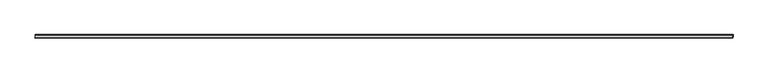
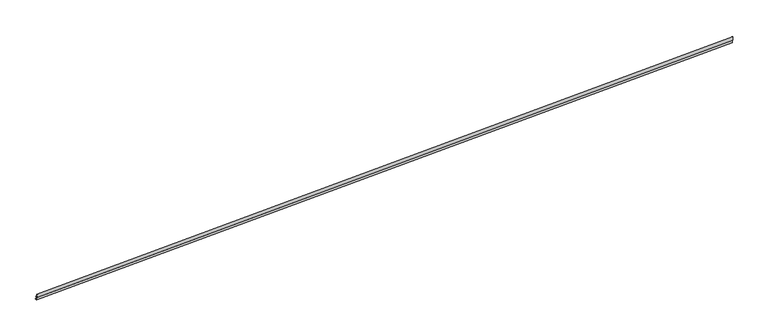
"""IFC4 building model written with IfcOpenShell, lengths in millimetres: proxy geometry, Generic Models 2:Generic Models 2:310765:Generic Models 2:310765 : Generic Models 2:Generic Models 2:310765:197 : Generic Models 2:Generic Models 2:310765:Generic Models 2:310765 : Generic Models 2:Generic Models 2:310765:300385."""

import ifcopenshell
import ifcopenshell.guid

model = None  # the IFC model being written
_history = None  # IfcOwnerHistory: only IFC2X3 demands one
_inside = {}  # id of a spatial element -> (the spatial element, [elements in it])
_under = {}  # id of a project, library or spatial element -> (it, [spatial elements below it])
_declared = {}  # id of a project -> (the project, [libraries it declares])
_typed = {}  # id of a type object -> (the type object, [elements of that type])
_made_of = {}  # id of a material, layer set ... -> (it, [elements and type objects made of it])


def new_model(schema):
    """Start an empty IFC model of exactly this schema.

    Asked for "IFC4X3", IfcOpenShell would pick the latest addendum, in which some entities
    have other attributes; the version numbers below select the first issue.
    IFC2X3 requires an IfcOwnerHistory on every rooted entity: one is made here for all.
    """
    global model, _history
    if schema == "IFC4X3":
        model = ifcopenshell.file(schema_version=(4, 3, 0, 0))
    else:
        model = ifcopenshell.file(schema=schema)
    _inside.clear()
    _under.clear()
    _declared.clear()
    _typed.clear()
    _made_of.clear()
    _history = None
    if model.schema == "IFC2X3":
        org = make("IfcOrganization", Name="unknown")
        user = make(
            "IfcPersonAndOrganization",
            ThePerson=make("IfcPerson", FamilyName="unknown"),
            TheOrganization=org,
        )
        app = make(
            "IfcApplication",
            ApplicationDeveloper=org,
            Version="unknown",
            ApplicationFullName="unknown",
            ApplicationIdentifier="unknown",
        )
        _history = make(
            "IfcOwnerHistory",
            OwningUser=user,
            OwningApplication=app,
            ChangeAction="ADDED",
            CreationDate=0,
        )
    return model


def make(cls, **values):
    """One entity of the class cls with the attributes given. An attribute that is None is left unset."""
    return model.create_entity(
        cls, **{name: value for name, value in values.items() if value is not None}
    )


def rooted(cls, **values):
    """An entity with a GlobalId (a new one), such as an element, a storey or a relation."""
    return make(cls, GlobalId=ifcopenshell.guid.new(), OwnerHistory=_history, **values)


def si_unit(unit_type, name, prefix=None):
    """IfcSIUnit, for example si_unit("LENGTHUNIT", "METRE", prefix="MILLI")."""
    return make("IfcSIUnit", UnitType=unit_type, Prefix=prefix, Name=name)


def assignment(units):
    """IfcUnitAssignment: the units of a project."""
    return None if units is None else make("IfcUnitAssignment", Units=units)


def point(xyz):
    """IfcCartesianPoint."""
    return None if xyz is None else make("IfcCartesianPoint", Coordinates=xyz)


def direction(xyz):
    """IfcDirection."""
    return None if xyz is None else make("IfcDirection", DirectionRatios=xyz)


def frame(location, z_axis=None, x_axis=None):
    """IfcAxis2Placement3D, a coordinate frame: its origin and axes. An axis left out is left unset."""
    return make(
        "IfcAxis2Placement3D",
        Location=point(location),
        Axis=direction(z_axis),
        RefDirection=direction(x_axis),
    )


def origin():
    """The frame at (0, 0, 0) with its axes left unset."""
    return frame((0.0, 0.0, 0.0))


def place(relative_to, where):
    """IfcLocalPlacement: puts the frame where relative to a parent placement (None: the world)."""
    return make(
        "IfcLocalPlacement", PlacementRelTo=relative_to, RelativePlacement=where
    )


def context(
    kind, dimensions, precision=None, world=None, true_north=None, identifier=None
):
    """IfcGeometricRepresentationContext, for example the 3D "Model" context."""
    return make(
        "IfcGeometricRepresentationContext",
        ContextIdentifier=identifier,
        ContextType=kind,
        CoordinateSpaceDimension=dimensions,
        Precision=precision,
        WorldCoordinateSystem=world,
        TrueNorth=true_north,
    )


def project(units=None, contexts=None):
    """IfcProject with its units and contexts."""
    return rooted(
        "IfcProject",
        Name="project",
        RepresentationContexts=contexts,
        UnitsInContext=assignment(units),
    )


def spatial(cls, under=None, at=None, **own):
    """A site, building, storey or space (cls), placed at a placement, below another one or the project."""
    s = rooted(cls, ObjectPlacement=at, **own)
    if under is not None:
        _under.setdefault(under.id(), (under, []))[1].append(s)
    return s


def polyline(points):
    """IfcPolyline through the points."""
    return make("IfcPolyline", Points=[point(p) for p in points])


def outline(outer, holes=None, kind="AREA"):
    """IfcArbitraryClosedProfileDef: a profile drawn as a closed curve; with holes, ...WithVoids."""
    if holes is None:
        return make("IfcArbitraryClosedProfileDef", ProfileType=kind, OuterCurve=outer)
    return make(
        "IfcArbitraryProfileDefWithVoids",
        ProfileType=kind,
        OuterCurve=outer,
        InnerCurves=holes,
    )


def extrude(swept, where, along, depth):
    """IfcExtrudedAreaSolid: the profile swept, set in the frame where, extruded along a direction by depth."""
    return make(
        "IfcExtrudedAreaSolid",
        SweptArea=swept,
        Position=where,
        ExtrudedDirection=direction(along),
        Depth=depth,
    )


def shape(context_of_items, identifier, shape_type, items):
    """IfcShapeRepresentation: the items that make up one representation, for example the "Body"."""
    return make(
        "IfcShapeRepresentation",
        ContextOfItems=context_of_items,
        RepresentationIdentifier=identifier,
        RepresentationType=shape_type,
        Items=items,
    )


def source(mapping_origin, context_of_items, identifier, shape_type, items):
    """IfcRepresentationMap: a shape defined once, which mapped items show again and again."""
    return make(
        "IfcRepresentationMap",
        MappingOrigin=mapping_origin,
        MappedRepresentation=shape(context_of_items, identifier, shape_type, items),
    )


def transform(
    local_origin,
    x_axis=None,
    y_axis=None,
    z_axis=None,
    scale=None,
    scale2=None,
    scale3=None,
    uniform=True,
):
    """IfcCartesianTransformationOperator3D, or its non-uniform kind. x_axis, y_axis, z_axis: its Axis1, 2, 3."""
    if uniform:
        return make(
            "IfcCartesianTransformationOperator3D",
            Axis1=direction(x_axis),
            Axis2=direction(y_axis),
            LocalOrigin=point(local_origin),
            Scale=scale,
            Axis3=direction(z_axis),
        )
    return make(
        "IfcCartesianTransformationOperator3DnonUniform",
        Axis1=direction(x_axis),
        Axis2=direction(y_axis),
        LocalOrigin=point(local_origin),
        Scale=scale,
        Axis3=direction(z_axis),
        Scale2=scale2,
        Scale3=scale3,
    )


def mapped(mapping_source, mapping_target):
    """IfcMappedItem: shows the shape of a source again, moved by a transform."""
    return make(
        "IfcMappedItem", MappingSource=mapping_source, MappingTarget=mapping_target
    )


def made_of(thing, what):
    """Note that an element or type object is made of a material, layer set ...; save() writes the relation."""
    if what is not None:
        _made_of.setdefault(what.id(), (what, []))[1].append(thing)
    return thing


def element(
    cls,
    number,
    at=None,
    inside=None,
    cuts=None,
    type_object=None,
    material=None,
    context=None,
    identifier="Body",
    shape_type=None,
    held_by="IfcProductDefinitionShape",
    body=None,
    shapes=None,
    **own,
):
    """One element of the class cls, such as IfcWall. Its Tag is "e" and its number.

    at: its placement. inside: the storey or other place that contains it. cuts: it is an
    opening in that element (IfcRelVoidsElement). A single representation is given by context,
    identifier, shape_type and body (its items); several are given by shapes. held_by: the class
    of the entity that holds the representations. save() writes the other relations.
    """
    e = rooted(cls, Tag="e%d" % number, ObjectPlacement=at, **own)
    if body is not None:
        shapes = [shape(context, identifier, shape_type, body)]
    if shapes is not None:
        e.Representation = make(held_by, Representations=shapes)
    if inside is not None:
        _inside.setdefault(inside.id(), (inside, []))[1].append(e)
    if cuts is not None:
        rooted(
            "IfcRelVoidsElement", RelatingBuildingElement=cuts, RelatedOpeningElement=e
        )
    if type_object is not None:
        _typed.setdefault(type_object.id(), (type_object, []))[1].append(e)
    return made_of(e, material)


def aggregate(whole, parts):
    """IfcRelAggregates: a whole, such as a stair, and the parts it consists of."""
    return rooted("IfcRelAggregates", RelatingObject=whole, RelatedObjects=parts)


def save(model, path):
    """Write the relations noted so far, then the file.

    IfcRelAggregates (storeys below a building ...), IfcRelContainedInSpatialStructure (elements
    in a storey), IfcRelDefinesByType, IfcRelAssociatesMaterial and IfcRelDeclares: one each for
    every whole, place, type object, material and project.
    """
    for whole, parts in _under.values():
        aggregate(whole, parts)
    for where, things in _inside.values():
        rooted(
            "IfcRelContainedInSpatialStructure",
            RelatedElements=things,
            RelatingStructure=where,
        )
    for kind, things in _typed.values():
        rooted("IfcRelDefinesByType", RelatedObjects=things, RelatingType=kind)
    for what, things in _made_of.values():
        rooted("IfcRelAssociatesMaterial", RelatedObjects=things, RelatingMaterial=what)
    for by, libraries in _declared.values():
        rooted("IfcRelDeclares", RelatingContext=by, RelatedDefinitions=libraries)
    model.write(path)


def generic_models_8b38b861(model_context):
    return source(origin(), model_context, "Body", "SweptSolid", [
        extrude(outline(polyline([(-6.35, 0.0), (-6.35, -90.4875), (-7.9375, -90.4875), (-7.9375, -1.5874999), (-72.095064, -1.5874999), (-72.095064, 11.1125), (-53.045064, 11.1125), (-53.045064, 9.5250001), (-70.507564, 9.5250001), (-70.507564, 0.0), (-6.35, 0.0)])), frame((560367.1930031, -578808.6038841, 4015.3424023), z_axis=(0.9991330730923568, 0.0, 0.04163054471206784), x_axis=(0.0, -1.0, 0.0)), (0.0, 0.0, 1.0), 18715.8200069),
        extrude(outline(polyline([(-48.7009311, 5.5562501), (-48.7009311, 56.35625), (-47.1134311, 56.35625), (-47.1134311, 3.96875), (-67.5700628, 3.96875), (-67.5700628, 5.5562501), (-48.7009311, 5.5562501)])), frame((560367.1930031, -578808.6038841, 4015.3424023), z_axis=(0.9991330730923568, 0.0, 0.04163054471206784), x_axis=(0.0, -1.0, 0.0)), (0.0, 0.0, 1.0), 18715.8200069),
        extrude(outline(polyline([(-36.5125, 89.69375), (-36.5125, 26.1937501), (-38.1, 26.1937501), (-38.1, 88.1062501), (-97.7325628, 88.1062501), (-97.7325628, 89.69375), (-36.5125, 89.69375)])), frame((560367.1930031, -578808.6038841, 4015.3424023), z_axis=(0.9991330730923568, 0.0, 0.04163054471206784), x_axis=(0.0, -1.0, 0.0)), (0.0, 0.0, 1.0), 18715.8200069),
    ])


if __name__ == "__main__":
    model = new_model("IFC4")
    model_context = context("Model", 3, world=origin())
    ifc_project = project(units=[si_unit("LENGTHUNIT", "METRE", prefix="MILLI")], contexts=[model_context])
    site = spatial("IfcSite", under=ifc_project)
    building = spatial("IfcBuilding", under=site)
    placement = place(None, origin())
    generic_models_shape = generic_models_8b38b861(model_context)
    element("IfcBuildingElementProxy", 1, Name="Generic Models 2:Generic Models 2:310765:Generic Models 2:310765 : Generic Models 2:Generic Models 2:310765:197 : Generic Models 2:Generic Models 2:310765:Generic Models 2:310765 : Generic Models 2:Generic Models 2:310765:300385", ObjectType="Generic Models 2:Generic Models 2:310765:Generic Models 2:310765 : Generic Models 2:Generic Models 2:310765:197 : Generic Models 2:Generic Models 2:310765:Generic Models 2:310765 : Generic Models 2:Generic Models 2:310765:300385", at=placement, inside=building, context=model_context, shape_type="MappedRepresentation", body=[
        mapped(generic_models_shape, transform((0.0, 0.0, 0.0), x_axis=(1.0, 0.0, 0.0), y_axis=(0.0, 1.0, 0.0), z_axis=(0.0, 0.0, 1.0))),
    ])
    save(model, "model.ifc")

# Revit data of these elements
# Type "Generic Models 2:Generic Models 2:310765:Generic Models 2:310765 : Generic Models 2:Generic Models 2:310765:197 : Generic Models 2:Generic Models 2:310765:Generic Models 2:310765 : Generic Models 2:Generic Models 2:310765:300385"
#   NameOverride = "Generic Models 2:Generic Models 2:310765:Generic Models 2:310765 : Generic Models 2:Generic Models 2:310765:300385"
#   ObjectTypeOverride = "Generic Models 2:310765 : Generic Models 2:Generic Models 2:310765"
#   Reference = "Generic Models 2"
#   Tag = "300385"
# Element 1 (IfcBuildingElementProxy, "Generic Models 2:Generic Models 2:310765:Generic Models 2:310765 : Generic Models 2:Generic Models 2:310765:197 : Generic Models 2:Generic Models 2:310765:Generic Models 2:310765 : Generic Models 2:Generic Models 2:310765:300385")
#   Materials on its faces: "BRAKE METAL COUNTERFLASHING"
# Materials
#   "BRAKE METAL COUNTERFLASHING": class "Unassigned", colour RGB 182 182 182, transparency 0, Cost = 0
